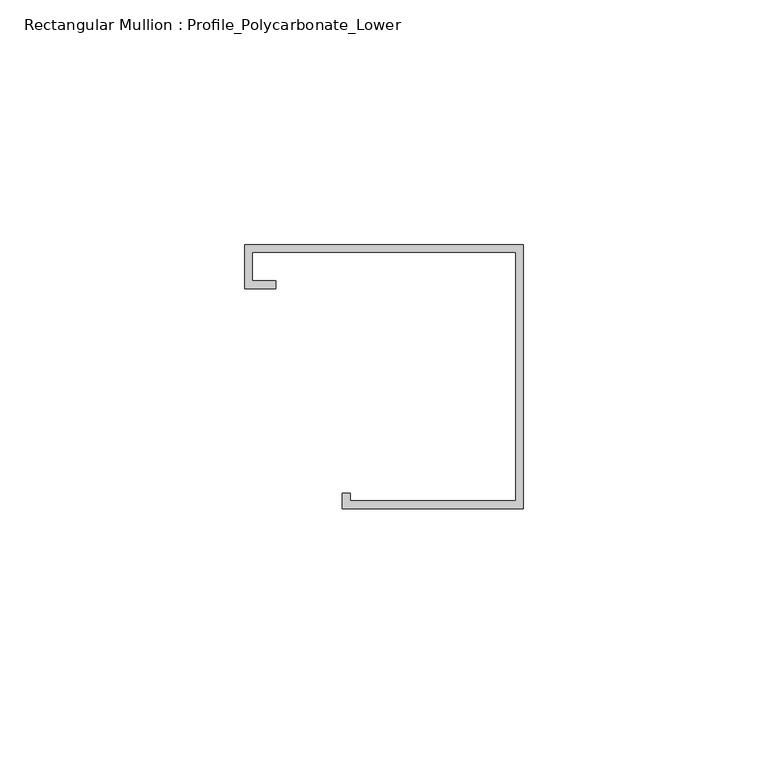
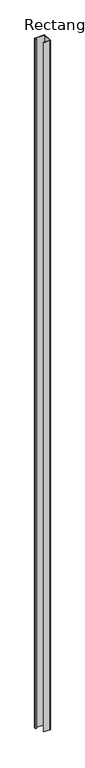
"""IFC4 building model written with IfcOpenShell, lengths in millimetres: member geometry, Rectangular Mullion : Profile_Polycarbonate_Lower."""

from ifc_helpers import new_model, si_unit, frame, origin, place, context, project, spatial, polyline, outline, extrude, source, transform, mapped, element, save


def rectangular_mullion_profile_polycarbonate_lower_07ae4ce1(model_context):
    return source(origin(), model_context, "Body", "SweptSolid", [
        extrude(outline(polyline([(0.0, 28.984575), (0.0, -25.015825), (-36.9824, -25.015825), (-36.9824, -21.840825), (-35.3949, -21.840825), (-35.3949, -23.428325), (-1.5875, -23.428325), (-1.5875, 27.397075), (-55.4101, 27.397075), (-55.4101, 21.580475), (-50.6476, 21.580475), (-50.6476, 19.992975), (-56.9976, 19.992975), (-56.9976, 28.984575), (0.0, 28.984575)])), frame((0.0, 0.0, -4116.6609733), z_axis=(0.0, 0.0, 1.0), x_axis=(1.0, 0.0, 0.0)), (0.0, 0.0, 1.0), 4116.6609733),
    ])


if __name__ == "__main__":
    model = new_model("IFC4")
    model_context = context("Model", 3, world=origin())
    ifc_project = project(units=[si_unit("LENGTHUNIT", "METRE", prefix="MILLI")], contexts=[model_context])
    site = spatial("IfcSite", under=ifc_project)
    building = spatial("IfcBuilding", under=site)
    placement = place(None, origin())
    rectangular_mullion_profile_polycarbonate_lower_shape = rectangular_mullion_profile_polycarbonate_lower_07ae4ce1(model_context)
    element("IfcMember", 1, ObjectType="Rectangular Mullion : Profile_Polycarbonate_Lower", at=placement, inside=building, context=model_context, shape_type="MappedRepresentation", body=[
        mapped(rectangular_mullion_profile_polycarbonate_lower_shape, transform((0.0, 0.0, 0.0), x_axis=(1.0, 0.0, 0.0), y_axis=(0.0, 1.0, 0.0), z_axis=(0.0, 0.0, 1.0))),
    ])
    save(model, "model.ifc")

# Revit data of these elements
# Type "Rectangular Mullion : Profile_Polycarbonate_Lower"
#   built-in parameter 1007322 = 0.177167 (stored number, unit not read)
#   built-in parameter 1007321 = 0 (stored number, unit not read)
#   built-in parameter 1007320 = 0.00520833 (stored number, unit not read)
